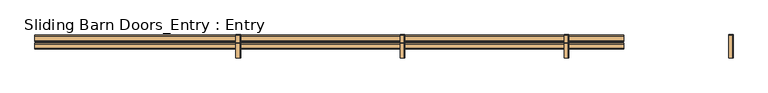
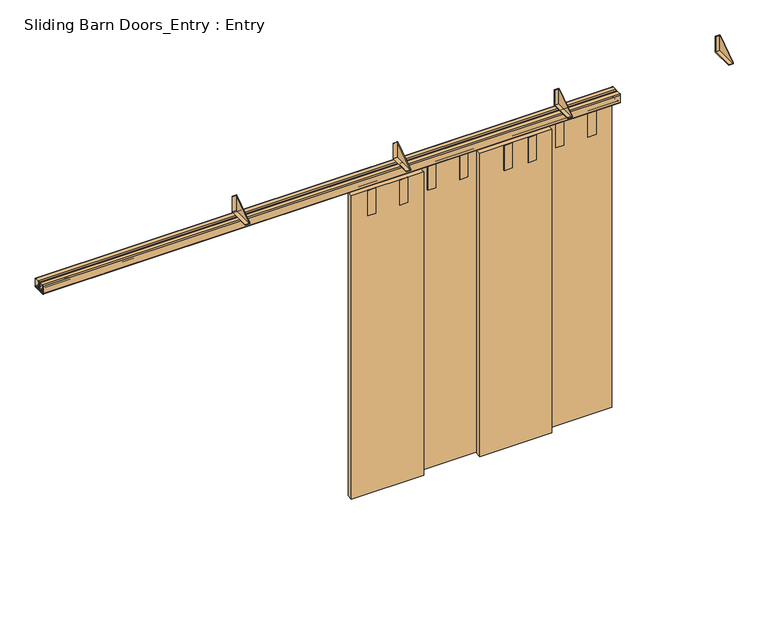
"""IFC4 building model written with IfcOpenShell, lengths in millimetres: door geometry, Sliding Barn Doors_Entry : Entry."""

from ifc_helpers import new_model, si_unit, point, frame, frame_2d, origin, place, context, project, spatial, polyline, circle_curve, trimmed, segment, composite_curve, outline, extrude, source, transform, mapped, element, save


def sliding_barn_doors_entry_entry_d8005735(model_context):
    return source(origin(), model_context, "Body", "SweptSolid", [
        extrude(outline(polyline([(-222.25, 2149.4037959), (-79.375, 2247.773), (-79.375, 2146.3), (-222.25, 2146.3), (-222.25, 2149.4037959)])), frame((521.1795573, 0.0, 0.0), z_axis=(1.0, 0.0, 0.0), x_axis=(0.0, 1.0, 0.0)), (0.0, 0.0, 1.0), 3.175),
        extrude(outline(polyline([(-76.2, 2143.125), (-222.25, 2143.125), (-222.25, 2146.3), (-79.375, 2146.3), (-79.375, 2247.773), (-76.2, 2247.773), (-76.2, 2143.125)])), frame((495.878776, 0.0, 0.0), z_axis=(1.0, 0.0, 0.0), x_axis=(0.0, 1.0, 0.0)), (0.0, 0.0, 1.0), 28.4757813),
        extrude(outline(polyline([(-222.25, 2149.4037959), (-79.375, 2247.773), (-79.375, 2146.3), (-222.25, 2146.3), (-222.25, 2149.4037959)])), frame((-499.053776, 0.0, 0.0), z_axis=(1.0, 0.0, 0.0), x_axis=(0.0, 1.0, 0.0)), (0.0, 0.0, 1.0), 3.175),
        extrude(outline(polyline([(-76.2, 2143.125), (-222.25, 2143.125), (-222.25, 2146.3), (-79.375, 2146.3), (-79.375, 2247.773), (-76.2, 2247.773), (-76.2, 2143.125)])), frame((-524.3545573, 0.0, 0.0), z_axis=(1.0, 0.0, 0.0), x_axis=(0.0, 1.0, 0.0)), (0.0, 0.0, 1.0), 28.4757813),
        extrude(outline(polyline([(-222.25, 2149.4037959), (-79.375, 2247.773), (-79.375, 2146.3), (-222.25, 2146.3), (-222.25, 2149.4037959)])), frame((-1519.2871094, 0.0, 0.0), z_axis=(1.0, 0.0, 0.0), x_axis=(0.0, 1.0, 0.0)), (0.0, 0.0, 1.0), 3.175),
        extrude(outline(polyline([(-76.2, 2143.125), (-222.25, 2143.125), (-222.25, 2146.3), (-79.375, 2146.3), (-79.375, 2247.773), (-76.2, 2247.773), (-76.2, 2143.125)])), frame((-1544.5878906, 0.0, 0.0), z_axis=(1.0, 0.0, 0.0), x_axis=(0.0, 1.0, 0.0)), (0.0, 0.0, 1.0), 28.4757812),
        extrude(outline(polyline([(-222.25, 2149.4037959), (-79.375, 2247.773), (-79.375, 2146.3), (-222.25, 2146.3), (-222.25, 2149.4037959)])), frame((1541.4128906, 0.0, 0.0), z_axis=(1.0, 0.0, 0.0), x_axis=(0.0, 1.0, 0.0)), (0.0, 0.0, 1.0), 3.175),
        extrude(outline(polyline([(-76.2, 2143.125), (-222.25, 2143.125), (-222.25, 2146.3), (-79.375, 2146.3), (-79.375, 2247.773), (-76.2, 2247.773), (-76.2, 2143.125)])), frame((1516.1121094, 0.0, 0.0), z_axis=(1.0, 0.0, 0.0), x_axis=(0.0, 1.0, 0.0)), (0.0, 0.0, 1.0), 28.4757812),
        extrude(outline(polyline([(-736.854, -165.1), (-736.854, -161.925), (-685.546, -161.925), (-685.546, -165.1), (-736.854, -165.1)])), frame((0.0, 0.0, 1889.252), z_axis=(0.0, 0.0, 1.0), x_axis=(1.0, 0.0, 0.0)), (0.0, 0.0, 1.0), 168.148),
        extrude(outline(polyline([(-533.654, -165.1), (-533.654, -161.925), (-482.346, -161.925), (-482.346, -165.1), (-533.654, -165.1)])), frame((0.0, 0.0, 1889.252), z_axis=(0.0, 0.0, 1.0), x_axis=(1.0, 0.0, 0.0)), (0.0, 0.0, 1.0), 168.148),
        extrude(outline(polyline([(-330.454, -117.475), (-330.454, -114.3), (-279.146, -114.3), (-279.146, -117.475), (-330.454, -117.475)])), frame((0.0, 0.0, 1889.252), z_axis=(0.0, 0.0, 1.0), x_axis=(1.0, 0.0, 0.0)), (0.0, 0.0, 1.0), 168.148),
        extrude(outline(polyline([(-127.254, -117.475), (-127.254, -114.3), (-75.946, -114.3), (-75.946, -117.475), (-127.254, -117.475)])), frame((0.0, 0.0, 1889.252), z_axis=(0.0, 0.0, 1.0), x_axis=(1.0, 0.0, 0.0)), (0.0, 0.0, 1.0), 168.148),
        extrude(outline(polyline([(126.746, -165.1), (126.746, -161.925), (178.054, -161.925), (178.054, -165.1), (126.746, -165.1)])), frame((0.0, 0.0, 1889.252), z_axis=(0.0, 0.0, 1.0), x_axis=(1.0, 0.0, 0.0)), (0.0, 0.0, 1.0), 168.148),
        extrude(outline(polyline([(279.146, -165.1), (279.146, -161.925), (330.454, -161.925), (330.454, -165.1), (279.146, -165.1)])), frame((0.0, 0.0, 1889.252), z_axis=(0.0, 0.0, 1.0), x_axis=(1.0, 0.0, 0.0)), (0.0, 0.0, 1.0), 168.148),
        extrude(outline(polyline([(482.346, -117.475), (482.346, -114.3), (533.654, -114.3), (533.654, -117.475), (482.346, -117.475)])), frame((0.0, 0.0, 1889.252), z_axis=(0.0, 0.0, 1.0), x_axis=(1.0, 0.0, 0.0)), (0.0, 0.0, 1.0), 168.148),
        extrude(outline(polyline([(685.546, -117.475), (685.546, -114.3), (736.854, -114.3), (736.854, -117.475), (685.546, -117.475)])), frame((0.0, 0.0, 1889.252), z_axis=(0.0, 0.0, 1.0), x_axis=(1.0, 0.0, 0.0)), (0.0, 0.0, 1.0), 168.148),
        extrude(outline(polyline([(-838.2, -161.925), (-838.2, -127.0), (-381.0, -127.0), (-381.0, -161.925), (-838.2, -161.925)])), frame((0.0, 0.0, 25.4), z_axis=(0.0, 0.0, 1.0), x_axis=(1.0, 0.0, 0.0)), (0.0, 0.0, 1.0), 2032.0),
        extrude(outline(polyline([(-25.4, -161.925), (-25.4, -127.0), (431.8, -127.0), (431.8, -161.925), (-25.4, -161.925)])), frame((0.0, 0.0, 25.4), z_axis=(0.0, 0.0, 1.0), x_axis=(1.0, 0.0, 0.0)), (0.0, 0.0, 1.0), 2032.0),
        extrude(outline(polyline([(-431.8, -114.3), (-431.8, -79.375), (25.4, -79.375), (25.4, -114.3), (-431.8, -114.3)])), frame((0.0, 0.0, 25.4), z_axis=(0.0, 0.0, 1.0), x_axis=(1.0, 0.0, 0.0)), (0.0, 0.0, 1.0), 2032.0),
        extrude(outline(polyline([(381.0, -114.3), (381.0, -79.375), (838.2, -79.375), (838.2, -114.3), (381.0, -114.3)])), frame((0.0, 0.0, 25.4), z_axis=(0.0, 0.0, 1.0), x_axis=(1.0, 0.0, 0.0)), (0.0, 0.0, 1.0), 2032.0),
        extrude(outline(composite_curve([segment(trimmed(circle_curve(frame_2d((-133.35, 2136.775)), 6.35), [point((-133.35, 2143.125))], [point((-127.0, 2136.775))], False, "CARTESIAN"), True, "CONTINUOUS"), segment(polyline([(-127.0, 2136.775), (-127.0, 2088.515)]), True, "CONTINUOUS"), segment(trimmed(circle_curve(frame_2d((-133.35, 2088.515)), 6.35), [point((-127.0, 2088.515))], [point((-133.35, 2082.165))], False, "CARTESIAN"), True, "CONTINUOUS"), segment(polyline([(-133.35, 2082.165), (-138.7586853, 2082.165)]), True, "CONTINUOUS"), segment(trimmed(circle_curve(frame_2d((-138.7586853, 2083.7525)), 1.5875), [point((-138.7586853, 2082.165))], [point((-140.3170184, 2083.4495907))], False, "CARTESIAN"), True, "CONTINUOUS"), segment(polyline([(-140.3170184, 2083.4495907), (-141.7425341, 2090.7832331), (-140.2263971, 2090.7832331), (-138.8404749, 2083.6532812), (-133.35, 2083.6532812)]), True, "CONTINUOUS"), segment(trimmed(circle_curve(frame_2d((-133.35, 2088.515)), 4.8617187), [point((-133.35, 2083.6532812))], [point((-128.4882813, 2088.515))], True, "CARTESIAN"), True, "CONTINUOUS"), segment(polyline([(-128.4882813, 2088.515), (-128.4882813, 2136.775)]), True, "CONTINUOUS"), segment(trimmed(circle_curve(frame_2d((-133.35, 2136.775)), 4.8617187), [point((-128.4882813, 2136.775))], [point((-133.35, 2141.6367187))], True, "CARTESIAN"), True, "CONTINUOUS"), segment(polyline([(-133.35, 2141.6367187), (-158.877, 2141.6367187)]), True, "CONTINUOUS"), segment(trimmed(circle_curve(frame_2d((-158.877, 2136.775)), 4.8617187), [point((-158.877, 2141.6367187))], [point((-163.7387188, 2136.775))], True, "CARTESIAN"), True, "CONTINUOUS"), segment(polyline([(-163.7387188, 2136.775), (-163.7387188, 2088.515)]), True, "CONTINUOUS"), segment(trimmed(circle_curve(frame_2d((-158.877, 2088.515)), 4.8617188), [point((-163.7387188, 2088.515))], [point((-158.877, 2083.6532812))], True, "CARTESIAN"), True, "CONTINUOUS"), segment(polyline([(-158.877, 2083.6532812), (-153.3865251, 2083.6532812), (-152.0006029, 2090.7832331), (-150.4844659, 2090.7832331), (-151.9099816, 2083.4495907)]), True, "CONTINUOUS"), segment(trimmed(circle_curve(frame_2d((-153.4683147, 2083.7525)), 1.5875), [point((-151.9099816, 2083.4495907))], [point((-153.4683147, 2082.165))], False, "CARTESIAN"), True, "CONTINUOUS"), segment(polyline([(-153.4683147, 2082.165), (-158.877, 2082.165)]), True, "CONTINUOUS"), segment(trimmed(circle_curve(frame_2d((-158.877, 2088.515)), 6.35), [point((-158.877, 2082.165))], [point((-165.227, 2088.515))], False, "CARTESIAN"), True, "CONTINUOUS"), segment(polyline([(-165.227, 2088.515), (-165.227, 2136.775)]), True, "CONTINUOUS"), segment(trimmed(circle_curve(frame_2d((-158.877, 2136.775)), 6.35), [point((-165.227, 2136.775))], [point((-158.877, 2143.125))], False, "CARTESIAN"), True, "CONTINUOUS"), segment(polyline([(-158.877, 2143.125), (-133.35, 2143.125)]), True, "CONTINUOUS")], self_intersect=False)), frame((-2794.0, 0.0, 0.0), z_axis=(1.0, 0.0, 0.0), x_axis=(0.0, 1.0, 0.0)), (0.0, 0.0, 1.0), 3657.6),
        extrude(outline(composite_curve([segment(trimmed(circle_curve(frame_2d((-85.725, 2136.775)), 6.35), [point((-85.725, 2143.125))], [point((-79.375, 2136.775))], False, "CARTESIAN"), True, "CONTINUOUS"), segment(polyline([(-79.375, 2136.775), (-79.375, 2088.515)]), True, "CONTINUOUS"), segment(trimmed(circle_curve(frame_2d((-85.725, 2088.515)), 6.35), [point((-79.375, 2088.515))], [point((-85.725, 2082.165))], False, "CARTESIAN"), True, "CONTINUOUS"), segment(polyline([(-85.725, 2082.165), (-91.1336853, 2082.165)]), True, "CONTINUOUS"), segment(trimmed(circle_curve(frame_2d((-91.1336853, 2083.7525)), 1.5875), [point((-91.1336853, 2082.165))], [point((-92.6920184, 2083.4495907))], False, "CARTESIAN"), True, "CONTINUOUS"), segment(polyline([(-92.6920184, 2083.4495907), (-94.1175341, 2090.7832331), (-92.6013971, 2090.7832331), (-91.2154749, 2083.6532812), (-85.725, 2083.6532812)]), True, "CONTINUOUS"), segment(trimmed(circle_curve(frame_2d((-85.725, 2088.515)), 4.8617187), [point((-85.725, 2083.6532812))], [point((-80.8632813, 2088.515))], True, "CARTESIAN"), True, "CONTINUOUS"), segment(polyline([(-80.8632813, 2088.515), (-80.8632813, 2136.775)]), True, "CONTINUOUS"), segment(trimmed(circle_curve(frame_2d((-85.725, 2136.775)), 4.8617187), [point((-80.8632813, 2136.775))], [point((-85.725, 2141.6367187))], True, "CARTESIAN"), True, "CONTINUOUS"), segment(polyline([(-85.725, 2141.6367187), (-111.252, 2141.6367187)]), True, "CONTINUOUS"), segment(trimmed(circle_curve(frame_2d((-111.252, 2136.775)), 4.8617187), [point((-111.252, 2141.6367187))], [point((-116.1137188, 2136.775))], True, "CARTESIAN"), True, "CONTINUOUS"), segment(polyline([(-116.1137188, 2136.775), (-116.1137188, 2088.515)]), True, "CONTINUOUS"), segment(trimmed(circle_curve(frame_2d((-111.252, 2088.515)), 4.8617187), [point((-116.1137188, 2088.515))], [point((-111.252, 2083.6532812))], True, "CARTESIAN"), True, "CONTINUOUS"), segment(polyline([(-111.252, 2083.6532812), (-105.7615251, 2083.6532812), (-104.3756029, 2090.7832331), (-102.8594659, 2090.7832331), (-104.2849816, 2083.4495907)]), True, "CONTINUOUS"), segment(trimmed(circle_curve(frame_2d((-105.8433147, 2083.7525)), 1.5875), [point((-104.2849816, 2083.4495907))], [point((-105.8433147, 2082.165))], False, "CARTESIAN"), True, "CONTINUOUS"), segment(polyline([(-105.8433147, 2082.165), (-111.252, 2082.165)]), True, "CONTINUOUS"), segment(trimmed(circle_curve(frame_2d((-111.252, 2088.515)), 6.35), [point((-111.252, 2082.165))], [point((-117.602, 2088.515))], False, "CARTESIAN"), True, "CONTINUOUS"), segment(polyline([(-117.602, 2088.515), (-117.602, 2136.775)]), True, "CONTINUOUS"), segment(trimmed(circle_curve(frame_2d((-111.252, 2136.775)), 6.35), [point((-117.602, 2136.775))], [point((-111.252, 2143.125))], False, "CARTESIAN"), True, "CONTINUOUS"), segment(polyline([(-111.252, 2143.125), (-85.725, 2143.125)]), True, "CONTINUOUS")], self_intersect=False)), frame((-2794.0, 0.0, 0.0), z_axis=(1.0, 0.0, 0.0), x_axis=(0.0, 1.0, 0.0)), (0.0, 0.0, 1.0), 3657.6),
    ])


if __name__ == "__main__":
    model = new_model("IFC4")
    model_context = context("Model", 3, world=origin())
    ifc_project = project(units=[si_unit("LENGTHUNIT", "METRE", prefix="MILLI")], contexts=[model_context])
    site = spatial("IfcSite", under=ifc_project)
    building = spatial("IfcBuilding", under=site)
    placement = place(None, origin())
    sliding_barn_doors_entry_entry_shape = sliding_barn_doors_entry_entry_d8005735(model_context)
    element("IfcDoor", 1, ObjectType="Sliding Barn Doors_Entry : Entry", at=placement, inside=building, context=model_context, shape_type="MappedRepresentation", body=[
        mapped(sliding_barn_doors_entry_entry_shape, transform((0.0, 0.0, 0.0), x_axis=(1.0, 0.0, 0.0), y_axis=(0.0, 1.0, 0.0), z_axis=(0.0, 0.0, 1.0))),
    ])
    save(model, "model.ifc")

# Revit data of these elements
# Type "Sliding Barn Doors_Entry : Entry"
#   Type Mark = "48"
#   OD_DS_Door_Type = "SLIDER"
#   Analytic Construction = "<None>"
#   rail_overlap_left = 0' - 1"
#   rail_length = 12' - 0"
#   overlap_left = 0' - 0"
#   overlap = 0' - 2"
#   bracket_right = 0' - 9"
#   bracket_left = 0' - 4"
#   Thickness = 0' - 1 3/8"
#   Panel Width = 1' - 6"
#   Panel Height = 6' - 8"
#   Gap 2 = 0' - 0 1/2"
#   Gap 1 = 0' - 0 7/8"
#   Frame Projection Ext. = 0' - 1"
#   Frame Projection Int. = 0' - 1"
#   Frame Width = 0' - 3"
#   Height = 6' - 5 3/8"
#   Width = 5' - 6"
#   Bracket_offset = 0' - 5"
#   Door_4 = yes
#   Door_3 = yes
#   Hardware Material = Metal - Aluminum
#   Door Material = Closet_1
#   Function = (empty or 0)
#   Wall Closure = (empty or 0)
# Element 1 (IfcDoor, "Sliding Barn Doors_Entry : Entry")
#   Materials on its faces: "Metal - Aluminum", "Closet_1"
# Materials
#   "Metal - Aluminum": class "Metal", colour RGB 247 247 247, transparency 0
#   "Closet_1": class "Paint", colour RGB 200 194 183, transparency 0, Cost = 0
